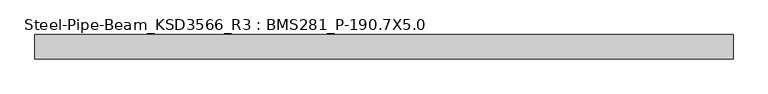
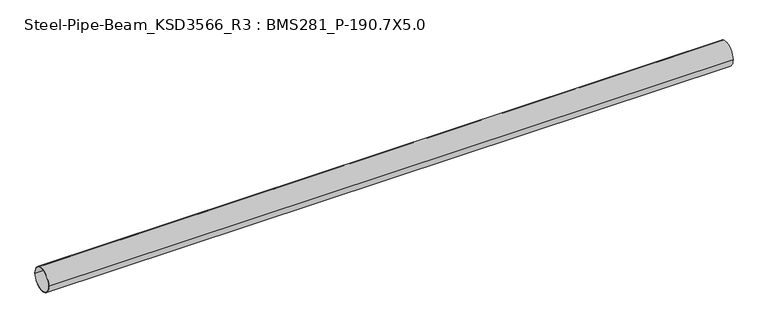
"""IFC4 building model written with IfcOpenShell, lengths in millimetres: member geometry, Steel-Pipe-Beam_KSD3566_R3 : BMS281_P-190.7X5.0."""

import ifcopenshell
import ifcopenshell.guid

model = None  # the IFC model being written
_history = None  # IfcOwnerHistory: only IFC2X3 demands one
_inside = {}  # id of a spatial element -> (the spatial element, [elements in it])
_under = {}  # id of a project, library or spatial element -> (it, [spatial elements below it])
_declared = {}  # id of a project -> (the project, [libraries it declares])
_typed = {}  # id of a type object -> (the type object, [elements of that type])
_made_of = {}  # id of a material, layer set ... -> (it, [elements and type objects made of it])


def new_model(schema):
    """Start an empty IFC model of exactly this schema.

    Asked for "IFC4X3", IfcOpenShell would pick the latest addendum, in which some entities
    have other attributes; the version numbers below select the first issue.
    IFC2X3 requires an IfcOwnerHistory on every rooted entity: one is made here for all.
    """
    global model, _history
    if schema == "IFC4X3":
        model = ifcopenshell.file(schema_version=(4, 3, 0, 0))
    else:
        model = ifcopenshell.file(schema=schema)
    _inside.clear()
    _under.clear()
    _declared.clear()
    _typed.clear()
    _made_of.clear()
    _history = None
    if model.schema == "IFC2X3":
        org = make("IfcOrganization", Name="unknown")
        user = make(
            "IfcPersonAndOrganization",
            ThePerson=make("IfcPerson", FamilyName="unknown"),
            TheOrganization=org,
        )
        app = make(
            "IfcApplication",
            ApplicationDeveloper=org,
            Version="unknown",
            ApplicationFullName="unknown",
            ApplicationIdentifier="unknown",
        )
        _history = make(
            "IfcOwnerHistory",
            OwningUser=user,
            OwningApplication=app,
            ChangeAction="ADDED",
            CreationDate=0,
        )
    return model


def make(cls, **values):
    """One entity of the class cls with the attributes given. An attribute that is None is left unset."""
    return model.create_entity(
        cls, **{name: value for name, value in values.items() if value is not None}
    )


def rooted(cls, **values):
    """An entity with a GlobalId (a new one), such as an element, a storey or a relation."""
    return make(cls, GlobalId=ifcopenshell.guid.new(), OwnerHistory=_history, **values)


def si_unit(unit_type, name, prefix=None):
    """IfcSIUnit, for example si_unit("LENGTHUNIT", "METRE", prefix="MILLI")."""
    return make("IfcSIUnit", UnitType=unit_type, Prefix=prefix, Name=name)


def assignment(units):
    """IfcUnitAssignment: the units of a project."""
    return None if units is None else make("IfcUnitAssignment", Units=units)


def point(xyz):
    """IfcCartesianPoint."""
    return None if xyz is None else make("IfcCartesianPoint", Coordinates=xyz)


def direction(xyz):
    """IfcDirection."""
    return None if xyz is None else make("IfcDirection", DirectionRatios=xyz)


def frame(location, z_axis=None, x_axis=None):
    """IfcAxis2Placement3D, a coordinate frame: its origin and axes. An axis left out is left unset."""
    return make(
        "IfcAxis2Placement3D",
        Location=point(location),
        Axis=direction(z_axis),
        RefDirection=direction(x_axis),
    )


def frame_2d(location, x_axis=None):
    """IfcAxis2Placement2D, a coordinate frame in the plane: its origin and x axis."""
    return make(
        "IfcAxis2Placement2D", Location=point(location), RefDirection=direction(x_axis)
    )


def origin():
    """The frame at (0, 0, 0) with its axes left unset."""
    return frame((0.0, 0.0, 0.0))


def origin_2d():
    """The frame at (0, 0) in the plane with its x axis left unset."""
    return frame_2d((0.0, 0.0))


def place(relative_to, where):
    """IfcLocalPlacement: puts the frame where relative to a parent placement (None: the world)."""
    return make(
        "IfcLocalPlacement", PlacementRelTo=relative_to, RelativePlacement=where
    )


def context(
    kind, dimensions, precision=None, world=None, true_north=None, identifier=None
):
    """IfcGeometricRepresentationContext, for example the 3D "Model" context."""
    return make(
        "IfcGeometricRepresentationContext",
        ContextIdentifier=identifier,
        ContextType=kind,
        CoordinateSpaceDimension=dimensions,
        Precision=precision,
        WorldCoordinateSystem=world,
        TrueNorth=true_north,
    )


def project(units=None, contexts=None):
    """IfcProject with its units and contexts."""
    return rooted(
        "IfcProject",
        Name="project",
        RepresentationContexts=contexts,
        UnitsInContext=assignment(units),
    )


def spatial(cls, under=None, at=None, **own):
    """A site, building, storey or space (cls), placed at a placement, below another one or the project."""
    s = rooted(cls, ObjectPlacement=at, **own)
    if under is not None:
        _under.setdefault(under.id(), (under, []))[1].append(s)
    return s


def circle_curve(where, radius):
    """IfcCircle in the frame where."""
    return make("IfcCircle", Position=where, Radius=radius)


def trimmed(basis, trim1, trim2, sense, master):
    """IfcTrimmedCurve: the piece of a basis curve between two trims."""
    return make(
        "IfcTrimmedCurve",
        BasisCurve=basis,
        Trim1=trim1,
        Trim2=trim2,
        SenseAgreement=sense,
        MasterRepresentation=master,
    )


def segment(curve, same_sense, transition):
    """IfcCompositeCurveSegment."""
    return make(
        "IfcCompositeCurveSegment",
        Transition=transition,
        SameSense=same_sense,
        ParentCurve=curve,
    )


def composite_curve(segments, self_intersect=None):
    """IfcCompositeCurve: segments joined end to end."""
    return make("IfcCompositeCurve", Segments=segments, SelfIntersect=self_intersect)


def outline(outer, holes=None, kind="AREA"):
    """IfcArbitraryClosedProfileDef: a profile drawn as a closed curve; with holes, ...WithVoids."""
    if holes is None:
        return make("IfcArbitraryClosedProfileDef", ProfileType=kind, OuterCurve=outer)
    return make(
        "IfcArbitraryProfileDefWithVoids",
        ProfileType=kind,
        OuterCurve=outer,
        InnerCurves=holes,
    )


def extrude(swept, where, along, depth):
    """IfcExtrudedAreaSolid: the profile swept, set in the frame where, extruded along a direction by depth."""
    return make(
        "IfcExtrudedAreaSolid",
        SweptArea=swept,
        Position=where,
        ExtrudedDirection=direction(along),
        Depth=depth,
    )


def shape(context_of_items, identifier, shape_type, items):
    """IfcShapeRepresentation: the items that make up one representation, for example the "Body"."""
    return make(
        "IfcShapeRepresentation",
        ContextOfItems=context_of_items,
        RepresentationIdentifier=identifier,
        RepresentationType=shape_type,
        Items=items,
    )


def source(mapping_origin, context_of_items, identifier, shape_type, items):
    """IfcRepresentationMap: a shape defined once, which mapped items show again and again."""
    return make(
        "IfcRepresentationMap",
        MappingOrigin=mapping_origin,
        MappedRepresentation=shape(context_of_items, identifier, shape_type, items),
    )


def transform(
    local_origin,
    x_axis=None,
    y_axis=None,
    z_axis=None,
    scale=None,
    scale2=None,
    scale3=None,
    uniform=True,
):
    """IfcCartesianTransformationOperator3D, or its non-uniform kind. x_axis, y_axis, z_axis: its Axis1, 2, 3."""
    if uniform:
        return make(
            "IfcCartesianTransformationOperator3D",
            Axis1=direction(x_axis),
            Axis2=direction(y_axis),
            LocalOrigin=point(local_origin),
            Scale=scale,
            Axis3=direction(z_axis),
        )
    return make(
        "IfcCartesianTransformationOperator3DnonUniform",
        Axis1=direction(x_axis),
        Axis2=direction(y_axis),
        LocalOrigin=point(local_origin),
        Scale=scale,
        Axis3=direction(z_axis),
        Scale2=scale2,
        Scale3=scale3,
    )


def mapped(mapping_source, mapping_target):
    """IfcMappedItem: shows the shape of a source again, moved by a transform."""
    return make(
        "IfcMappedItem", MappingSource=mapping_source, MappingTarget=mapping_target
    )


def made_of(thing, what):
    """Note that an element or type object is made of a material, layer set ...; save() writes the relation."""
    if what is not None:
        _made_of.setdefault(what.id(), (what, []))[1].append(thing)
    return thing


def element(
    cls,
    number,
    at=None,
    inside=None,
    cuts=None,
    type_object=None,
    material=None,
    context=None,
    identifier="Body",
    shape_type=None,
    held_by="IfcProductDefinitionShape",
    body=None,
    shapes=None,
    **own,
):
    """One element of the class cls, such as IfcWall. Its Tag is "e" and its number.

    at: its placement. inside: the storey or other place that contains it. cuts: it is an
    opening in that element (IfcRelVoidsElement). A single representation is given by context,
    identifier, shape_type and body (its items); several are given by shapes. held_by: the class
    of the entity that holds the representations. save() writes the other relations.
    """
    e = rooted(cls, Tag="e%d" % number, ObjectPlacement=at, **own)
    if body is not None:
        shapes = [shape(context, identifier, shape_type, body)]
    if shapes is not None:
        e.Representation = make(held_by, Representations=shapes)
    if inside is not None:
        _inside.setdefault(inside.id(), (inside, []))[1].append(e)
    if cuts is not None:
        rooted(
            "IfcRelVoidsElement", RelatingBuildingElement=cuts, RelatedOpeningElement=e
        )
    if type_object is not None:
        _typed.setdefault(type_object.id(), (type_object, []))[1].append(e)
    return made_of(e, material)


def aggregate(whole, parts):
    """IfcRelAggregates: a whole, such as a stair, and the parts it consists of."""
    return rooted("IfcRelAggregates", RelatingObject=whole, RelatedObjects=parts)


def save(model, path):
    """Write the relations noted so far, then the file.

    IfcRelAggregates (storeys below a building ...), IfcRelContainedInSpatialStructure (elements
    in a storey), IfcRelDefinesByType, IfcRelAssociatesMaterial and IfcRelDeclares: one each for
    every whole, place, type object, material and project.
    """
    for whole, parts in _under.values():
        aggregate(whole, parts)
    for where, things in _inside.values():
        rooted(
            "IfcRelContainedInSpatialStructure",
            RelatedElements=things,
            RelatingStructure=where,
        )
    for kind, things in _typed.values():
        rooted("IfcRelDefinesByType", RelatedObjects=things, RelatingType=kind)
    for what, things in _made_of.values():
        rooted("IfcRelAssociatesMaterial", RelatedObjects=things, RelatingMaterial=what)
    for by, libraries in _declared.values():
        rooted("IfcRelDeclares", RelatingContext=by, RelatedDefinitions=libraries)
    model.write(path)


def steel_pipe_beam_ksd3566_r3_bms281_p_190_7x5_0_c00e4b08(model_context):
    return source(origin(), model_context, "Body", "SweptSolid", [
        extrude(outline(composite_curve([segment(trimmed(circle_curve(origin_2d(), 95.35), [point((-95.35, 0.0))], [point((95.35, 0.0))], False, "CARTESIAN"), True, "CONTINUOUS"), segment(trimmed(circle_curve(origin_2d(), 95.35), [point((95.35, 0.0))], [point((-95.35, 0.0))], False, "CARTESIAN"), True, "CONTINUOUS")], self_intersect=False), holes=[composite_curve([segment(trimmed(circle_curve(origin_2d(), 90.35), [point((90.35, 0.0))], [point((-90.35, 0.0))], True, "CARTESIAN"), True, "CONTINUOUS"), segment(trimmed(circle_curve(origin_2d(), 90.35), [point((-90.35, 0.0))], [point((90.35, 0.0))], True, "CARTESIAN"), True, "CONTINUOUS")], self_intersect=False)]), frame((-2752.4445734, 0.0, 0.0), z_axis=(1.0, 0.0, 0.0), x_axis=(0.0, 1.0, 0.0)), (0.0, 0.0, 1.0), 5477.7690397),
    ])


if __name__ == "__main__":
    model = new_model("IFC4")
    model_context = context("Model", 3, world=origin())
    ifc_project = project(units=[si_unit("LENGTHUNIT", "METRE", prefix="MILLI")], contexts=[model_context])
    site = spatial("IfcSite", under=ifc_project)
    building = spatial("IfcBuilding", under=site)
    placement = place(None, origin())
    steel_pipe_beam_ksd3566_r3_bms281_p_190_7x5_0_shape = steel_pipe_beam_ksd3566_r3_bms281_p_190_7x5_0_c00e4b08(model_context)
    element("IfcMember", 1, ObjectType="Steel-Pipe-Beam_KSD3566_R3 : BMS281_P-190.7X5.0", at=placement, inside=building, context=model_context, shape_type="MappedRepresentation", body=[
        mapped(steel_pipe_beam_ksd3566_r3_bms281_p_190_7x5_0_shape, transform((0.0, 0.0, 0.0), x_axis=(1.0, 0.0, 0.0), y_axis=(0.0, 1.0, 0.0), z_axis=(0.0, 0.0, 1.0))),
    ])
    save(model, "model.ifc")

# Revit data of these elements
# Type "Steel-Pipe-Beam_KSD3566_R3 : BMS281_P-190.7X5.0"
#   Keynote = "P-190.7X5.0"
#   SteelWeight = "Light"
#   t = 0.0050 m
#   Surface Area = 0.599102 m²/m
#   Section Area = 29.1697 cm²
#   Mass per Unit Length = 22.8982 kg/m
#   Length [instance default] = 1.5000 m
#   D = 0.1907 m
#   hec_material4 [instance default] = none
#   hec_material3 [instance default] = none
#   hec_material2 [instance default] = none
#   hec_material1 [instance default] = none
#   Structural Material [instance default] = Steel, 45-345
#   Assembly Code = ""
# Element 1 (IfcMember, "Steel-Pipe-Beam_KSD3566_R3 : BMS281_P-190.7X5.0")
#   Structural Material = none
# Materials
#   "Steel, 45-345": class "Metal", colour RGB 189 187 185, transparency 0, Description = "Steel 345 MPa", Cost = 0
